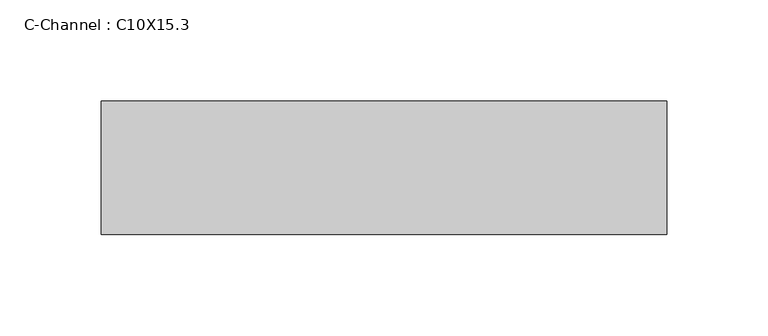
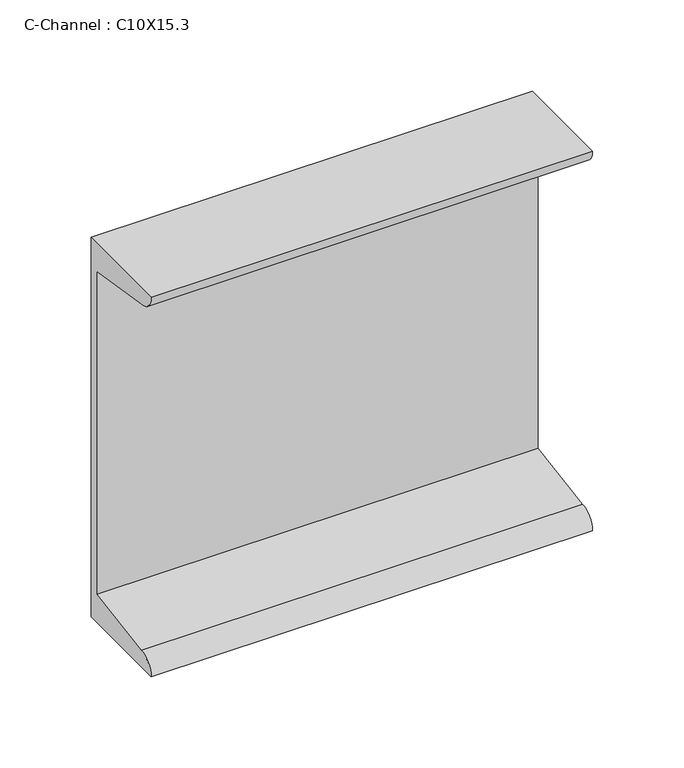
"""IFC4 building model written with IfcOpenShell, lengths in millimetres: beam geometry, C-Channel : C10X15.3."""

from ifc_helpers import new_model, si_unit, point, frame, frame_2d, origin, place, context, project, spatial, polyline, circle_curve, trimmed, segment, composite_curve, outline, extrude, source, transform, mapped, element, save


def c_channel_c10x15_3_669d7114(model_context):
    return source(origin(), model_context, "Body", "SweptSolid", [
        extrude(outline(composite_curve([segment(polyline([(16.1036, 127.0), (16.1036, -127.0), (-49.9364, -127.0)]), True, "CONTINUOUS"), segment(trimmed(circle_curve(frame_2d((-38.862, -127.0)), 11.0744), [point((-49.9364, -127.0))], [point((-38.862, -115.9256))], False, "CARTESIAN"), True, "CONTINUOUS"), segment(polyline([(-38.862, -115.9256), (10.0076, -108.1854158), (10.0076, 108.1854158), (-38.862, 115.9256)]), True, "CONTINUOUS"), segment(trimmed(circle_curve(frame_2d((-38.862, 127.0)), 11.0744), [point((-38.862, 115.9256))], [point((-49.9364, 127.0))], False, "CARTESIAN"), True, "CONTINUOUS"), segment(polyline([(-49.9364, 127.0), (16.1036, 127.0)]), True, "CONTINUOUS")], self_intersect=False)), frame((-127.0, 0.0, 0.0), z_axis=(1.0, 0.0, 0.0), x_axis=(0.0, 1.0, 0.0)), (0.0, 0.0, 1.0), 279.4),
    ])


if __name__ == "__main__":
    model = new_model("IFC4")
    model_context = context("Model", 3, world=origin())
    ifc_project = project(units=[si_unit("LENGTHUNIT", "METRE", prefix="MILLI")], contexts=[model_context])
    site = spatial("IfcSite", under=ifc_project)
    building = spatial("IfcBuilding", under=site)
    placement = place(None, origin())
    c_channel_c10x15_3_shape = c_channel_c10x15_3_669d7114(model_context)
    element("IfcBeam", 1, ObjectType="C-Channel : C10X15.3", at=placement, inside=building, context=model_context, shape_type="MappedRepresentation", body=[
        mapped(c_channel_c10x15_3_shape, transform((0.0, 0.0, 0.0), x_axis=(1.0, 0.0, 0.0), y_axis=(0.0, 1.0, 0.0), z_axis=(0.0, 0.0, 1.0))),
    ])
    save(model, "model.ifc")

# Revit data of these elements
# Type "C-Channel : C10X15.3"
#   Assembly Code = "B10"
#   W = 15.3
#   Length [instance default] = 5' - 0"
#   bf = 0' - 2.6"
#   d = 0' - 10"
#   tf = 0' - 0.436"
#   tw = 0' - 0.24"
#   x = 0' - 0.634"
#   A = 0.0311111 SF
#   Structural Material [instance default] = Steel ASTM A36
# Element 1 (IfcBeam, "C-Channel : C10X15.3")
#   Structural Material = Steel ASTM A992
#   Materials on its faces: "Steel ASTM A992"
# Materials
#   "Steel ASTM A36": class "Metal", colour RGB 199 199 199, transparency 0, Description = "Structural steel, ASTM A36 Grade B, mill finish", Cost = 0
#   "Steel ASTM A992": class "Metal", colour RGB 199 199 199, transparency 0, Description = "Structural steel 50ksi", Cost = 0
